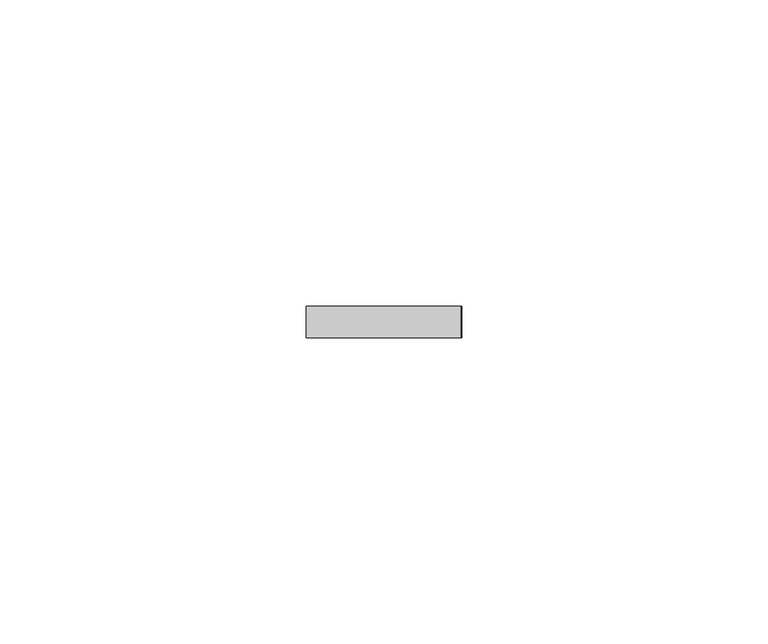
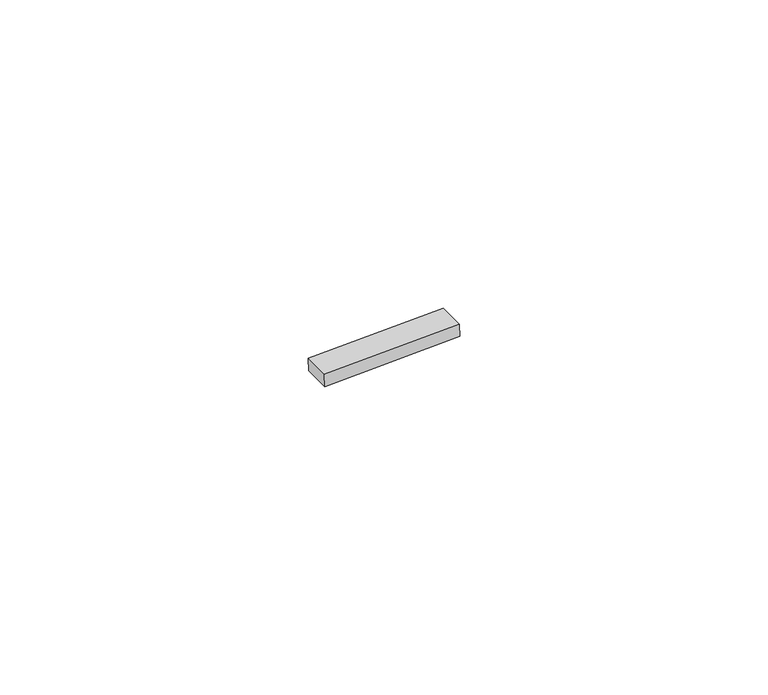
"""IFC4 building model written with IfcOpenShell, lengths in millimetres: proxy geometry, Inner panel:Inner panel:1:Inner panel:1 : Inner panel:Inner panel:300324:2:Inner panel:1:Inner panel:1 : Inner panel:Inner panel:300324:2 : Inner panel:Inner panel:1:Inner panel:1 : Inner panel:Inner panel:300324:300043:172 : Inner panel:Inner panel:1:Inner panel:1 : Inner panel:Inner panel:300324:2:Inner panel:1:Inner panel:1 : Inner panel:Inner panel:300324:2 : Inner panel:Inner panel:1:Inner panel:1 : Inner panel:Inner panel:300324:300043:308120."""

from ifc_helpers import new_model, si_unit, frame, origin, place, context, project, spatial, polyline, outline, extrude, source, transform, mapped, element, save


def generic_models_4f8dff8d(model_context):
    return source(origin(), model_context, "Body", "SweptSolid", [
        extrude(outline(polyline([(0.0, -25.4), (0.0, 0.0), (5.213809, 0.0), (5.213809, -25.4), (0.0, -25.4)])), frame((560380.9331581, -564994.107991, 3950.5346612), z_axis=(-0.041630544712223896, 0.0, 0.9991330730923502), x_axis=(0.0, -1.0, 0.0)), (0.0, 0.0, 1.0), 2.4763745),
    ])


if __name__ == "__main__":
    model = new_model("IFC4")
    model_context = context("Model", 3, world=origin())
    ifc_project = project(units=[si_unit("LENGTHUNIT", "METRE", prefix="MILLI")], contexts=[model_context])
    site = spatial("IfcSite", under=ifc_project)
    building = spatial("IfcBuilding", under=site)
    placement = place(None, origin())
    generic_models_shape = generic_models_4f8dff8d(model_context)
    element("IfcBuildingElementProxy", 1, Name="Inner panel:Inner panel:1:Inner panel:1 : Inner panel:Inner panel:300324:2:Inner panel:1:Inner panel:1 : Inner panel:Inner panel:300324:2 : Inner panel:Inner panel:1:Inner panel:1 : Inner panel:Inner panel:300324:300043:172 : Inner panel:Inner panel:1:Inner panel:1 : Inner panel:Inner panel:300324:2:Inner panel:1:Inner panel:1 : Inner panel:Inner panel:300324:2 : Inner panel:Inner panel:1:Inner panel:1 : Inner panel:Inner panel:300324:300043:308120", ObjectType="Inner panel:Inner panel:1:Inner panel:1 : Inner panel:Inner panel:300324:2:Inner panel:1:Inner panel:1 : Inner panel:Inner panel:300324:2 : Inner panel:Inner panel:1:Inner panel:1 : Inner panel:Inner panel:300324:300043:172 : Inner panel:Inner panel:1:Inner panel:1 : Inner panel:Inner panel:300324:2:Inner panel:1:Inner panel:1 : Inner panel:Inner panel:300324:2 : Inner panel:Inner panel:1:Inner panel:1 : Inner panel:Inner panel:300324:300043:308120", at=placement, inside=building, context=model_context, shape_type="MappedRepresentation", body=[
        mapped(generic_models_shape, transform((0.0, 0.0, 0.0), x_axis=(1.0, 0.0, 0.0), y_axis=(0.0, 1.0, 0.0), z_axis=(0.0, 0.0, 1.0))),
    ])
    save(model, "model.ifc")

# Revit data of these elements
# Type "Inner panel:Inner panel:1:Inner panel:1 : Inner panel:Inner panel:300324:2:Inner panel:1:Inner panel:1 : Inner panel:Inner panel:300324:2 : Inner panel:Inner panel:1:Inner panel:1 : Inner panel:Inner panel:300324:300043:172 : Inner panel:Inner panel:1:Inner panel:1 : Inner panel:Inner panel:300324:2:Inner panel:1:Inner panel:1 : Inner panel:Inner panel:300324:2 : Inner panel:Inner panel:1:Inner panel:1 : Inner panel:Inner panel:300324:300043:308120"
#   NameOverride = "Inner panel:Inner panel:1:Inner panel:1 : Inner panel:Inner panel:300324:2:Inner panel:1:Inner panel:1 : Inner panel:Inner panel:300324:2 : Inner panel:Inner panel:1:Inner panel:1 : Inner panel:Inner panel:300324:300043:308120"
#   ObjectTypeOverride = "Inner panel:1:Inner panel:1 : Inner panel:Inner panel:300324:2 : Inner panel:Inner panel:1:Inner panel:1 : Inner panel:Inner panel:300324:300043"
#   Reference = "Inner panel"
#   Tag = "308120"
# Element 1 (IfcBuildingElementProxy, "Inner panel:Inner panel:1:Inner panel:1 : Inner panel:Inner panel:300324:2:Inner panel:1:Inner panel:1 : Inner panel:Inner panel:300324:2 : Inner panel:Inner panel:1:Inner panel:1 : Inner panel:Inner panel:300324:300043:172 : Inner panel:Inner panel:1:Inner panel:1 : Inner panel:Inner panel:300324:2:Inner panel:1:Inner panel:1 : Inner panel:Inner panel:300324:2 : Inner panel:Inner panel:1:Inner panel:1 : Inner panel:Inner panel:300324:300043:308120")
#   Materials on its faces: "AT CLIP - 1\" WIDE NON ABSORBENT, WEATHER-RESISTANT NEOPRENE/EPDM/SBR FOAM"
# Materials
#   "AT CLIP - 1\" WIDE NON ABSORBENT, WEATHER-RESISTANT NEOPRENE/EPDM/SBR FOAM": class "Generic", colour RGB 85 85 85, transparency 0, Cost = 0
